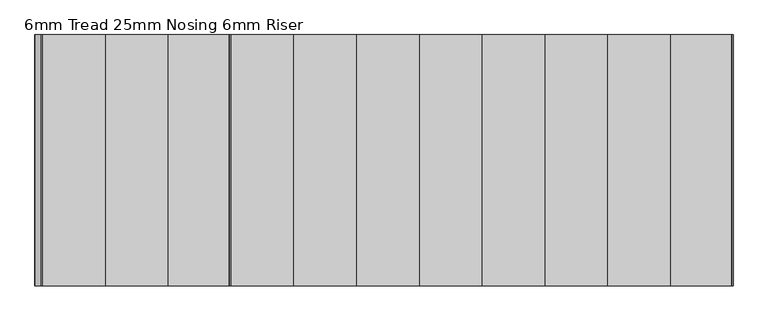
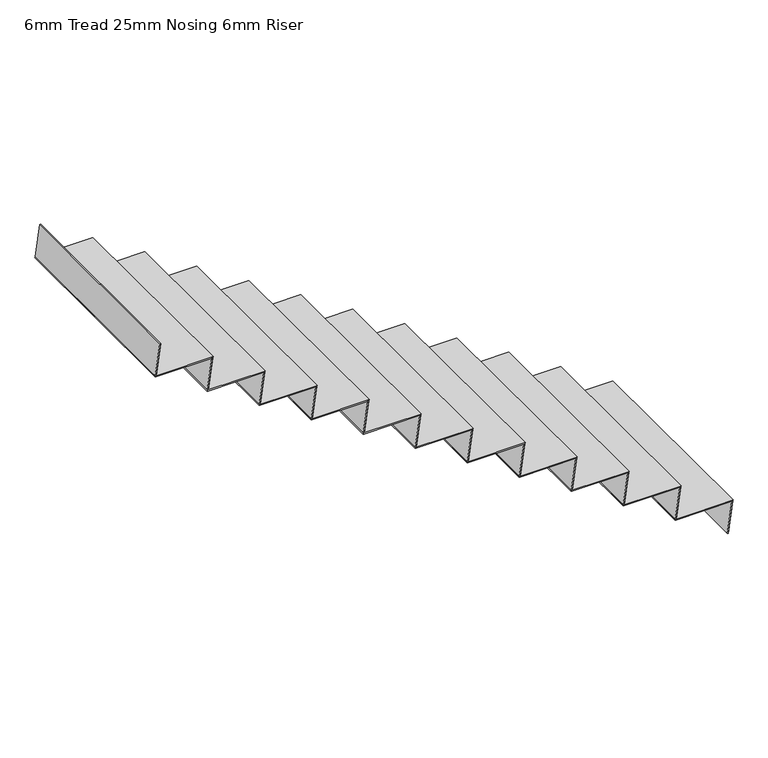
"""IFC4 building model written with IfcOpenShell, lengths in millimetres: stair flight geometry, 6mm Tread 25mm Nosing 6mm Riser."""

from ifc_helpers import new_model, si_unit, origin, place, context, project, spatial, faceted_brep, source, transform, mapped, element, save


def stair_flight_6mm_tread_25mm_nosing_6mm_riser_97df853b(model_context):
    return source(origin(), model_context, "Body", "Brep", [
        faceted_brep([(-13631.0599092, 11395.4345331, 24411.7647059), (-13631.9099092, 11395.4345331, 24405.7647059), (-13631.9099092, 10295.4345331, 24405.7647059), (-13631.0599092, 10295.4345331, 24411.7647059), (-13325.0, 10295.4345331, 24411.7647059), (-13325.0, 11395.4345331, 24411.7647059), (-13325.85, 11395.4345331, 24405.7647059), (-13325.85, 10295.4345331, 24405.7647059)], [[[0, 1, 2, 3]], [[3, 4, 5, 0]], [[2, 1, 6, 7]], [[4, 3, 2, 7]], [[0, 5, 6, 1]], [[5, 4, 7, 6]]]),
        faceted_brep([(-13325.85, 11395.4345331, 24405.7647059), (-13350.0, 11395.4345331, 24235.2941176), (-13356.0599092, 11395.4345331, 24235.2941176), (-13331.9099092, 11395.4345331, 24405.7647059), (-13325.85, 10295.4345331, 24405.7647059), (-13331.9099092, 10295.4345331, 24405.7647059), (-13356.0599092, 10295.4345331, 24235.2941176), (-13350.0, 10295.4345331, 24235.2941176)], [[[0, 1, 2, 3]], [[4, 5, 6, 7]], [[1, 0, 4, 7]], [[2, 1, 7, 6]], [[3, 2, 6, 5]], [[0, 3, 5, 4]]]),
        faceted_brep([(-13600.85, 11395.4345331, 24582.2352941), (-13625.0, 11395.4345331, 24411.7647059), (-13631.0599092, 11395.4345331, 24411.7647059), (-13606.9099092, 11395.4345331, 24582.2352941), (-13600.85, 10295.4345331, 24582.2352941), (-13606.9099092, 10295.4345331, 24582.2352941), (-13631.0599092, 10295.4345331, 24411.7647059), (-13625.0, 10295.4345331, 24411.7647059)], [[[0, 1, 2, 3]], [[4, 5, 6, 7]], [[1, 0, 4, 7]], [[2, 1, 7, 6]], [[3, 2, 6, 5]], [[0, 3, 5, 4]]]),
        faceted_brep([(-13906.0599092, 10295.4345331, 24588.2352941), (-13600.0, 10295.4345331, 24588.2352941), (-13600.0, 11395.4345331, 24588.2352941), (-13906.0599092, 11395.4345331, 24588.2352941), (-13906.9099092, 10295.4345331, 24582.2352941), (-13906.9099092, 11395.4345331, 24582.2352941), (-13600.85, 11395.4345331, 24582.2352941), (-13600.85, 10295.4345331, 24582.2352941)], [[[0, 1, 2, 3]], [[4, 5, 6, 7]], [[1, 0, 4, 7]], [[3, 2, 6, 5]], [[3, 5, 4, 0]], [[2, 1, 7, 6]]]),
        faceted_brep([(-13875.85, 11395.4345331, 24758.7058824), (-13900.0, 11395.4345331, 24588.2352941), (-13906.0599092, 11395.4345331, 24588.2352941), (-13881.9099092, 11395.4345331, 24758.7058824), (-13875.85, 10295.4345331, 24758.7058824), (-13881.9099092, 10295.4345331, 24758.7058824), (-13906.0599092, 10295.4345331, 24588.2352941), (-13900.0, 10295.4345331, 24588.2352941)], [[[0, 1, 2, 3]], [[4, 5, 6, 7]], [[1, 0, 4, 7]], [[2, 1, 7, 6]], [[3, 2, 6, 5]], [[0, 3, 5, 4]]]),
        faceted_brep([(-14181.0599092, 10295.4345331, 24764.7058824), (-13875.0, 10295.4345331, 24764.7058824), (-13875.0, 11395.4345331, 24764.7058824), (-14181.0599092, 11395.4345331, 24764.7058824), (-14181.9099092, 10295.4345331, 24758.7058824), (-14181.9099092, 11395.4345331, 24758.7058824), (-13875.85, 11395.4345331, 24758.7058824), (-13875.85, 10295.4345331, 24758.7058824)], [[[0, 1, 2, 3]], [[4, 5, 6, 7]], [[1, 0, 4, 7]], [[3, 2, 6, 5]], [[3, 5, 4, 0]], [[2, 1, 7, 6]]]),
        faceted_brep([(-14150.85, 11395.4345331, 24935.1764706), (-14175.0, 11395.4345331, 24764.7058824), (-14181.0599092, 11395.4345331, 24764.7058824), (-14156.9099092, 11395.4345331, 24935.1764706), (-14150.85, 10295.4345331, 24935.1764706), (-14156.9099092, 10295.4345331, 24935.1764706), (-14181.0599092, 10295.4345331, 24764.7058824), (-14175.0, 10295.4345331, 24764.7058824)], [[[0, 1, 2, 3]], [[4, 5, 6, 7]], [[1, 0, 4, 7]], [[2, 1, 7, 6]], [[3, 2, 6, 5]], [[0, 3, 5, 4]]]),
        faceted_brep([(-14456.0599092, 10295.4345331, 24941.1764706), (-14150.0, 10295.4345331, 24941.1764706), (-14150.0, 11395.4345331, 24941.1764706), (-14456.0599092, 11395.4345331, 24941.1764706), (-14456.9099092, 10295.4345331, 24935.1764706), (-14456.9099092, 11395.4345331, 24935.1764706), (-14150.85, 11395.4345331, 24935.1764706), (-14150.85, 10295.4345331, 24935.1764706)], [[[0, 1, 2, 3]], [[4, 5, 6, 7]], [[1, 0, 4, 7]], [[3, 2, 6, 5]], [[3, 5, 4, 0]], [[2, 1, 7, 6]]]),
        faceted_brep([(-14425.85, 11395.4345331, 25111.6470588), (-14450.0, 11395.4345331, 24941.1764706), (-14456.0599092, 11395.4345331, 24941.1764706), (-14431.9099092, 11395.4345331, 25111.6470588), (-14425.85, 10295.4345331, 25111.6470588), (-14431.9099092, 10295.4345331, 25111.6470588), (-14456.0599092, 10295.4345331, 24941.1764706), (-14450.0, 10295.4345331, 24941.1764706)], [[[0, 1, 2, 3]], [[4, 5, 6, 7]], [[1, 0, 4, 7]], [[2, 1, 7, 6]], [[3, 2, 6, 5]], [[0, 3, 5, 4]]]),
        faceted_brep([(-14731.0599092, 10295.4345331, 25117.6470588), (-14425.0, 10295.4345331, 25117.6470588), (-14425.0, 11395.4345331, 25117.6470588), (-14731.0599092, 11395.4345331, 25117.6470588), (-14731.9099092, 10295.4345331, 25111.6470588), (-14731.9099092, 11395.4345331, 25111.6470588), (-14425.85, 11395.4345331, 25111.6470588), (-14425.85, 10295.4345331, 25111.6470588)], [[[0, 1, 2, 3]], [[4, 5, 6, 7]], [[1, 0, 4, 7]], [[3, 2, 6, 5]], [[3, 5, 4, 0]], [[2, 1, 7, 6]]]),
        faceted_brep([(-14700.85, 11395.4345331, 25288.1176471), (-14725.0, 11395.4345331, 25117.6470588), (-14731.0599092, 11395.4345331, 25117.6470588), (-14706.9099092, 11395.4345331, 25288.1176471), (-14700.85, 10295.4345331, 25288.1176471), (-14706.9099092, 10295.4345331, 25288.1176471), (-14731.0599092, 10295.4345331, 25117.6470588), (-14725.0, 10295.4345331, 25117.6470588)], [[[0, 1, 2, 3]], [[4, 5, 6, 7]], [[1, 0, 4, 7]], [[2, 1, 7, 6]], [[3, 2, 6, 5]], [[0, 3, 5, 4]]]),
        faceted_brep([(-15006.0599092, 10295.4345331, 25294.1176471), (-14700.0, 10295.4345331, 25294.1176471), (-14700.0, 11395.4345331, 25294.1176471), (-15006.0599092, 11395.4345331, 25294.1176471), (-15006.9099092, 10295.4345331, 25288.1176471), (-15006.9099092, 11395.4345331, 25288.1176471), (-14700.85, 11395.4345331, 25288.1176471), (-14700.85, 10295.4345331, 25288.1176471)], [[[0, 1, 2, 3]], [[4, 5, 6, 7]], [[1, 0, 4, 7]], [[3, 2, 6, 5]], [[3, 5, 4, 0]], [[2, 1, 7, 6]]]),
        faceted_brep([(-14975.85, 11395.4345331, 25464.5882353), (-15000.0, 11395.4345331, 25294.1176471), (-15006.0599092, 11395.4345331, 25294.1176471), (-14981.9099092, 11395.4345331, 25464.5882353), (-14975.85, 10295.4345331, 25464.5882353), (-14981.9099092, 10295.4345331, 25464.5882353), (-15006.0599092, 10295.4345331, 25294.1176471), (-15000.0, 10295.4345331, 25294.1176471)], [[[0, 1, 2, 3]], [[4, 5, 6, 7]], [[1, 0, 4, 7]], [[2, 1, 7, 6]], [[3, 2, 6, 5]], [[0, 3, 5, 4]]]),
        faceted_brep([(-15281.0599092, 10295.4345331, 25470.5882353), (-14975.0, 10295.4345331, 25470.5882353), (-14975.0, 11395.4345331, 25470.5882353), (-15281.0599092, 11395.4345331, 25470.5882353), (-15281.9099092, 10295.4345331, 25464.5882353), (-15281.9099092, 11395.4345331, 25464.5882353), (-14975.85, 11395.4345331, 25464.5882353), (-14975.85, 10295.4345331, 25464.5882353)], [[[0, 1, 2, 3]], [[4, 5, 6, 7]], [[1, 0, 4, 7]], [[3, 2, 6, 5]], [[3, 5, 4, 0]], [[2, 1, 7, 6]]]),
        faceted_brep([(-15250.85, 11395.4345331, 25641.0588235), (-15275.0, 11395.4345331, 25470.5882353), (-15281.0599092, 11395.4345331, 25470.5882353), (-15256.9099092, 11395.4345331, 25641.0588235), (-15250.85, 10295.4345331, 25641.0588235), (-15256.9099092, 10295.4345331, 25641.0588235), (-15281.0599092, 10295.4345331, 25470.5882353), (-15275.0, 10295.4345331, 25470.5882353)], [[[0, 1, 2, 3]], [[4, 5, 6, 7]], [[1, 0, 4, 7]], [[2, 1, 7, 6]], [[3, 2, 6, 5]], [[0, 3, 5, 4]]]),
        faceted_brep([(-15556.0599092, 10295.4345331, 25647.0588235), (-15250.0, 10295.4345331, 25647.0588235), (-15250.0, 11395.4345331, 25647.0588235), (-15556.0599092, 11395.4345331, 25647.0588235), (-15556.9099092, 10295.4345331, 25641.0588235), (-15556.9099092, 11395.4345331, 25641.0588235), (-15250.85, 11395.4345331, 25641.0588235), (-15250.85, 10295.4345331, 25641.0588235)], [[[0, 1, 2, 3]], [[4, 5, 6, 7]], [[1, 0, 4, 7]], [[3, 2, 6, 5]], [[3, 5, 4, 0]], [[2, 1, 7, 6]]]),
        faceted_brep([(-15525.85, 11395.4345331, 25817.5294118), (-15550.0, 11395.4345331, 25647.0588235), (-15556.0599092, 11395.4345331, 25647.0588235), (-15531.9099092, 11395.4345331, 25817.5294118), (-15525.85, 10295.4345331, 25817.5294118), (-15531.9099092, 10295.4345331, 25817.5294118), (-15556.0599092, 10295.4345331, 25647.0588235), (-15550.0, 10295.4345331, 25647.0588235)], [[[0, 1, 2, 3]], [[4, 5, 6, 7]], [[1, 0, 4, 7]], [[2, 1, 7, 6]], [[3, 2, 6, 5]], [[0, 3, 5, 4]]]),
        faceted_brep([(-15831.0599092, 10295.4345331, 25823.5294118), (-15525.0, 10295.4345331, 25823.5294118), (-15525.0, 11395.4345331, 25823.5294118), (-15831.0599092, 11395.4345331, 25823.5294118), (-15831.9099092, 10295.4345331, 25817.5294118), (-15831.9099092, 11395.4345331, 25817.5294118), (-15525.85, 11395.4345331, 25817.5294118), (-15525.85, 10295.4345331, 25817.5294118)], [[[0, 1, 2, 3]], [[4, 5, 6, 7]], [[1, 0, 4, 7]], [[3, 2, 6, 5]], [[3, 5, 4, 0]], [[2, 1, 7, 6]]]),
        faceted_brep([(-15800.85, 11395.4345331, 25994.0), (-15825.0, 11395.4345331, 25823.5294118), (-15831.0599092, 11395.4345331, 25823.5294118), (-15806.9099092, 11395.4345331, 25994.0), (-15800.85, 10295.4345331, 25994.0), (-15806.9099092, 10295.4345331, 25994.0), (-15831.0599092, 10295.4345331, 25823.5294118), (-15825.0, 10295.4345331, 25823.5294118)], [[[0, 1, 2, 3]], [[4, 5, 6, 7]], [[1, 0, 4, 7]], [[2, 1, 7, 6]], [[3, 2, 6, 5]], [[0, 3, 5, 4]]]),
        faceted_brep([(-16106.0599092, 10295.4345331, 26000.0), (-15800.0, 10295.4345331, 26000.0), (-15800.0, 11395.4345331, 26000.0), (-16106.0599092, 11395.4345331, 26000.0), (-16106.9099092, 10295.4345331, 25994.0), (-16106.9099092, 11395.4345331, 25994.0), (-15800.85, 11395.4345331, 25994.0), (-15800.85, 10295.4345331, 25994.0)], [[[0, 1, 2, 3]], [[4, 5, 6, 7]], [[1, 0, 4, 7]], [[3, 2, 6, 5]], [[3, 5, 4, 0]], [[2, 1, 7, 6]]]),
        faceted_brep([(-16350.85, 11395.4345331, 26346.9411765), (-16375.0, 11395.4345331, 26176.4705882), (-16381.0599092, 11395.4345331, 26176.4705882), (-16356.9099092, 11395.4345331, 26346.9411765), (-16350.85, 10295.4345331, 26346.9411765), (-16356.9099092, 10295.4345331, 26346.9411765), (-16381.0599092, 10295.4345331, 26176.4705882), (-16375.0, 10295.4345331, 26176.4705882)], [[[0, 1, 2, 3]], [[4, 5, 6, 7]], [[1, 0, 4, 7]], [[2, 1, 7, 6]], [[3, 2, 6, 5]], [[0, 3, 5, 4]]]),
        faceted_brep([(-16075.85, 11395.4345331, 26170.4705882), (-16100.0, 11395.4345331, 26000.0), (-16106.0599092, 11395.4345331, 26000.0), (-16081.9099092, 11395.4345331, 26170.4705882), (-16075.85, 10295.4345331, 26170.4705882), (-16081.9099092, 10295.4345331, 26170.4705882), (-16106.0599092, 10295.4345331, 26000.0), (-16100.0, 10295.4345331, 26000.0)], [[[0, 1, 2, 3]], [[4, 5, 6, 7]], [[1, 0, 4, 7]], [[2, 1, 7, 6]], [[3, 2, 6, 5]], [[0, 3, 5, 4]]]),
        faceted_brep([(-16381.0599092, 10295.4345331, 26176.4705882), (-16350.0, 10295.4345331, 26176.4705882), (-16075.0, 10295.4345331, 26176.4705882), (-16075.0, 11395.4345331, 26176.4705882), (-16381.0599092, 11395.4345331, 26176.4705882), (-16381.9099092, 10295.4345331, 26170.4705882), (-16381.9099092, 11395.4345331, 26170.4705882), (-16075.85, 11395.4345331, 26170.4705882), (-16075.85, 10295.4345331, 26170.4705882), (-16350.0, 10295.4345331, 26170.4705882)], [[[0, 1, 2, 3, 4]], [[5, 6, 7, 8, 9]], [[1, 0, 5, 9]], [[2, 1, 9, 8]], [[4, 3, 7, 6]], [[4, 6, 5, 0]], [[3, 2, 8, 7]]]),
    ])


if __name__ == "__main__":
    model = new_model("IFC4")
    model_context = context("Model", 3, world=origin())
    ifc_project = project(units=[si_unit("LENGTHUNIT", "METRE", prefix="MILLI")], contexts=[model_context])
    site = spatial("IfcSite", under=ifc_project)
    building = spatial("IfcBuilding", under=site)
    placement = place(None, origin())
    stair_flight_6mm_tread_25mm_nosing_6mm_riser_shape = stair_flight_6mm_tread_25mm_nosing_6mm_riser_97df853b(model_context)
    element("IfcStairFlight", 1, ObjectType="6mm Tread 25mm Nosing 6mm Riser", at=placement, inside=building, context=model_context, shape_type="MappedRepresentation", body=[
        mapped(stair_flight_6mm_tread_25mm_nosing_6mm_riser_shape, transform((0.0, 0.0, 0.0), x_axis=(1.0, 0.0, 0.0), y_axis=(0.0, 1.0, 0.0), z_axis=(0.0, 0.0, 1.0))),
    ])
    save(model, "model.ifc")

# Revit data of these elements
# Element 1 (IfcStairFlight, "6mm Tread 25mm Nosing 6mm Riser")
#   Materials on its faces: "Steel, Paint Finish, Dark Gray"
# Materials
#   "Steel, Paint Finish, Dark Gray": class "Metal", colour RGB 89 89 89, transparency 0, Description = "Steel, paint finish, dark gray, glossy", Cost = 0
